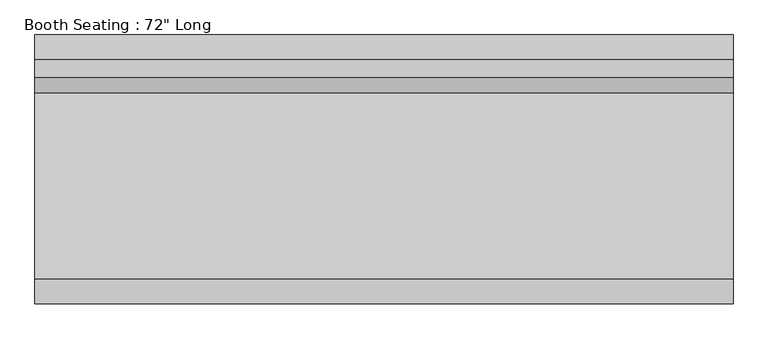
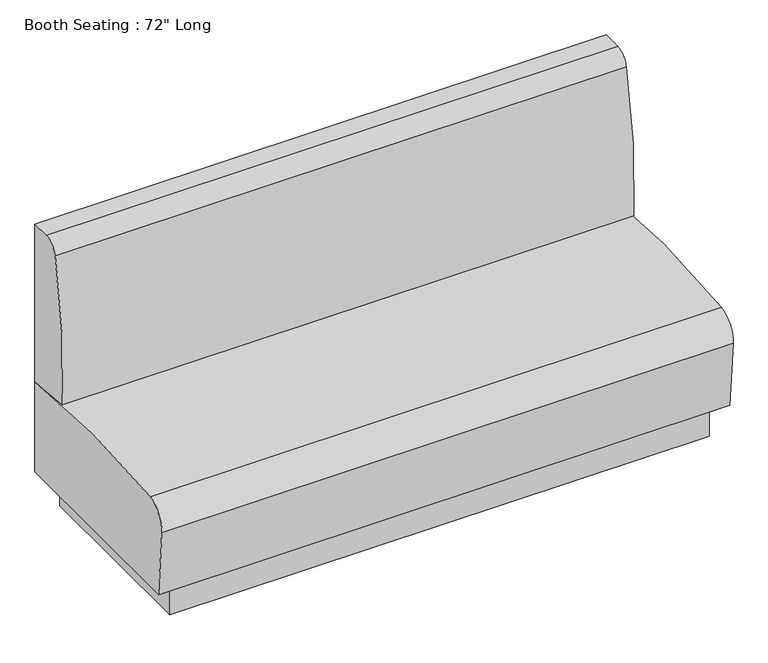
"""IFC4 building model written with IfcOpenShell, lengths in millimetres: furniture geometry."""

from ifc_helpers import new_model, si_unit, point, frame, frame_2d, origin, origin_with_axes, place, context, project, spatial, polyline, circle_curve, trimmed, segment, composite_curve, outline, extrude, source, transform, mapped, element, save


def furniture_e9c3bc78(model_context):
    return source(origin(), model_context, "Body", "SweptSolid", [
        extrude(outline(composite_curve([segment(polyline([(355.6, 939.8), (355.6, 406.4), (203.2, 420.809063)]), True, "CONTINUOUS"), segment(trimmed(circle_curve(frame_2d((1896.6191414, 522.5154157)), 1696.4706218), [point((203.2, 420.809063))], [point((242.7504703, 900.3129667))], False, "CARTESIAN"), True, "CONTINUOUS"), segment(trimmed(circle_curve(frame_2d((292.2747753, 889.0)), 50.8), [point((242.7504703, 900.3129667))], [point((292.2747753, 939.8))], False, "CARTESIAN"), True, "CONTINUOUS"), segment(polyline([(292.2747753, 939.8), (355.6, 939.8)]), True, "CONTINUOUS")], self_intersect=False)), frame((-914.4, 0.0, 0.0), z_axis=(1.0, 0.0, 0.0), x_axis=(0.0, 1.0, 0.0)), (0.0, 0.0, 1.0), 1828.8),
        extrude(outline(composite_curve([segment(trimmed(circle_curve(frame_2d((-272.6641824, 328.7396957)), 76.2), [point((-348.6009692, 322.4116302))], [point((-282.6626275, 404.2808838))], False, "CARTESIAN"), True, "CONTINUOUS"), segment(trimmed(circle_curve(frame_2d((44.6835428, -2068.9155338)), 2494.7657275), [point((-282.6626275, 404.2808838))], [point((355.6, 406.4))], False, "CARTESIAN"), True, "CONTINUOUS"), segment(polyline([(355.6, 406.4), (355.6, 101.6), (-330.2, 101.6), (-348.6009692, 322.4116302)]), True, "CONTINUOUS")], self_intersect=False)), frame((-914.4, 0.0, 0.0), z_axis=(1.0, 0.0, 0.0), x_axis=(0.0, 1.0, 0.0)), (0.0, 0.0, 1.0), 1828.8),
        extrude(outline(polyline([(863.6, 304.8), (863.6, -304.8), (-863.6, -304.8), (-863.6, 304.8), (863.6, 304.8)])), origin_with_axes(), (0.0, 0.0, 1.0), 101.6),
    ])


if __name__ == "__main__":
    model = new_model("IFC4")
    model_context = context("Model", 3, world=origin())
    ifc_project = project(units=[si_unit("LENGTHUNIT", "METRE", prefix="MILLI")], contexts=[model_context])
    site = spatial("IfcSite", under=ifc_project)
    building = spatial("IfcBuilding", under=site)
    placement = place(None, origin())
    furniture_shape = furniture_e9c3bc78(model_context)
    element("IfcFurniture", 1, ObjectType="Booth Seating : 72\" Long", at=placement, inside=building, context=model_context, shape_type="MappedRepresentation", body=[
        mapped(furniture_shape, transform((0.0, 0.0, 0.0), x_axis=(1.0, 0.0, 0.0), y_axis=(0.0, 1.0, 0.0), z_axis=(0.0, 0.0, 1.0))),
    ])
    save(model, "model.ifc")

# Revit data of these elements
# Type "Booth Seating : 72\" Long"
#   Type Mark = "SB2"
#   Seat Height = 1' - 4"
#   Length = 6' - 0"
#   Depth = 2' - 4"
#   Back Height = 3' - 1"
#   Number of Persons = 3
#   Default Elevation = 0
# Element 1 (IfcFurniture, "Booth Seating : 72\" Long")
#   Materials on its faces: "Leather, Dark Brown", "Plastic, Opaque Black"
# Materials
#   "Leather, Dark Brown": class "Textile", colour RGB 57 45 39, transparency 0, Description = "Leather, dark brown", Cost = 0
#   "Plastic, Opaque Black": class "Plastic", colour RGB 5 5 5, transparency 0, Description = "Plastic, generic, opaque black", Cost = 0
